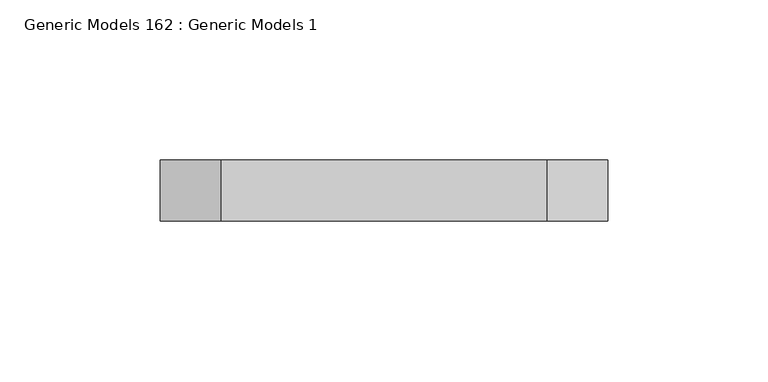
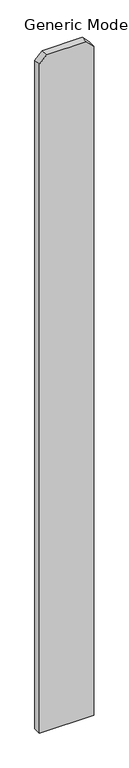
"""IFC4 building model written with IfcOpenShell, lengths in millimetres: proxy geometry, Generic Models 162 : Generic Models 1."""

from ifc_helpers import new_model, si_unit, frame, origin, place, context, project, spatial, polyline, outline, extrude, source, transform, mapped, element, save


def generic_models_162_generic_models_1_249433e1(model_context):
    return source(origin(), model_context, "Body", "SweptSolid", [
        extrude(outline(polyline([(76.2, 54684.6125), (1885.95, 54684.6125), (1905.0, 54665.5625), (1905.0, 54563.9625), (1885.95, 54544.9125), (76.2, 54544.9125), (76.2, 54684.6125)])), frame((0.0, 547.6875, 0.0), z_axis=(0.0, 1.0, 0.0), x_axis=(0.0, 0.0, 1.0)), (0.0, 0.0, 1.0), 19.05),
    ])


if __name__ == "__main__":
    model = new_model("IFC4")
    model_context = context("Model", 3, world=origin())
    ifc_project = project(units=[si_unit("LENGTHUNIT", "METRE", prefix="MILLI")], contexts=[model_context])
    site = spatial("IfcSite", under=ifc_project)
    building = spatial("IfcBuilding", under=site)
    placement = place(None, origin())
    generic_models_162_generic_models_1_shape = generic_models_162_generic_models_1_249433e1(model_context)
    element("IfcBuildingElementProxy", 1, Name="Generic Models 162 : Generic Models 1", ObjectType="Generic Models 162 : Generic Models 1", at=placement, inside=building, context=model_context, shape_type="MappedRepresentation", body=[
        mapped(generic_models_162_generic_models_1_shape, transform((0.0, 0.0, 0.0), x_axis=(1.0, 0.0, 0.0), y_axis=(0.0, 1.0, 0.0), z_axis=(0.0, 0.0, 1.0))),
    ])
    save(model, "model.ifc")

# Revit data of these elements
# Element 1 (IfcBuildingElementProxy, "Generic Models 162 : Generic Models 1")
#   Materials on its faces: "VERTICAL 1X6 CEDAR PLANKS W/ CLEAR WOOD SEALER"
# Materials
#   "VERTICAL 1X6 CEDAR PLANKS W/ CLEAR WOOD SEALER": class "Wood", colour RGB 234 198 147, transparency 0, Description = "Pinus Echinata", Cost = 0
